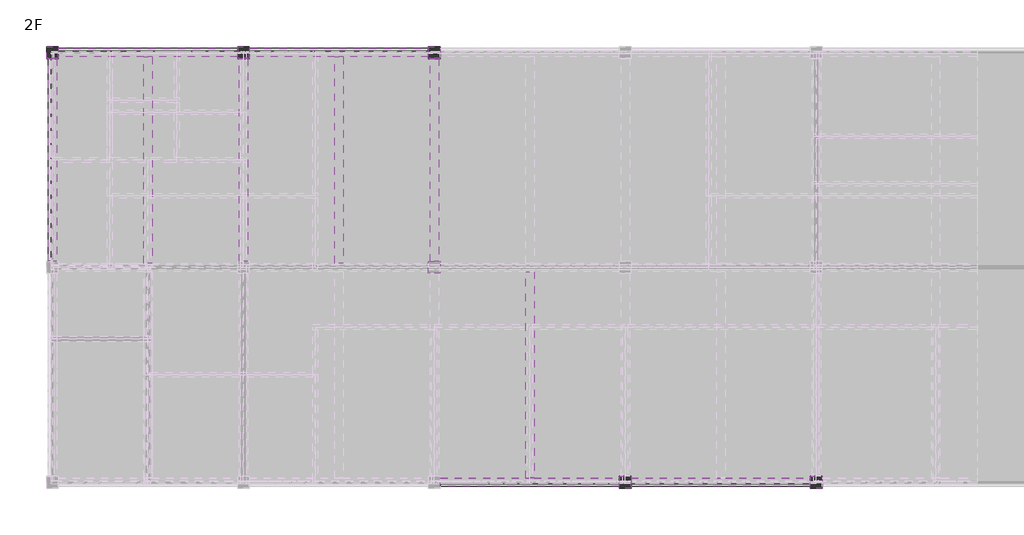
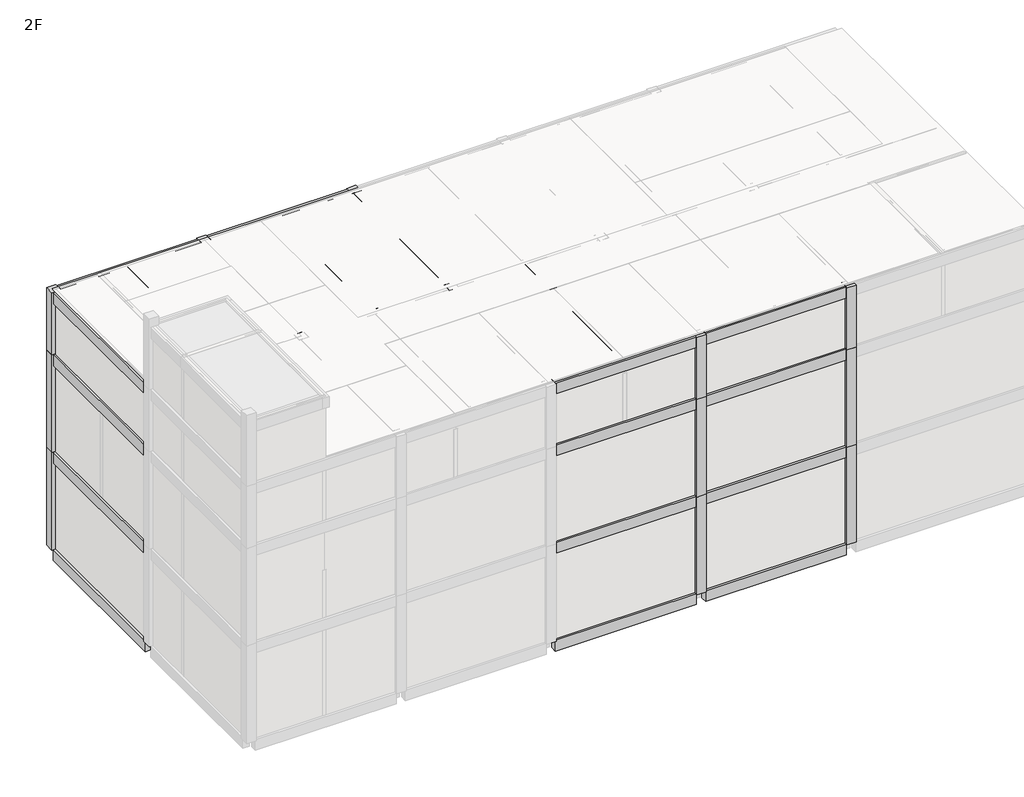
# One storey, part 5 of 7: 40 beams, 17 columns.
"""IFC4 building model written with IfcOpenShell, lengths in millimetres."""

from ifc_helpers import new_model, si_unit, frame, origin, place, context, project, spatial, polyline, outline, extrude, faceted_brep, element, save

model = new_model("IFC4")

# Units and contexts
model_context = context("Model", 3, world=origin())
ifc_project = project(units=[si_unit("LENGTHUNIT", "METRE", prefix="MILLI")], contexts=[model_context])

# Site, building, storey
site = spatial("IfcSite", under=ifc_project)
building = spatial("IfcBuilding", under=site)
storey = spatial("IfcBuildingStorey", under=building, Name="2F", Elevation=3500.0)

# Beams
placement = place(None, origin())
element("IfcBeam", 1, ObjectType="Concrete-Rectangular-Beam : BM111_400x500_RG1", at=placement, inside=storey, context=model_context, shape_type="SweptSolid", body=[
    extrude(outline(polyline([(49284.6521483, 181748.8614395), (49634.6521483, 181748.8614395), (49634.6521483, 173098.8614395), (49284.6521483, 173098.8614395), (49284.6521483, 181748.8614395)])), frame((0.0, 0.0, 2900.0), z_axis=(0.0, 0.0, 1.0), x_axis=(1.0, 0.0, 0.0)), (0.0, 0.0, 1.0), 600.0),
])
element("IfcBeam", 2, ObjectType="Concrete-Rectangular-Beam : BM111_400x500_RG1", at=placement, inside=storey, context=model_context, shape_type="SweptSolid", body=[
    extrude(outline(polyline([(57634.6521483, 173098.8614395), (57284.6521483, 173098.8614395), (57284.6521483, 181748.8614395), (57634.6521483, 181748.8614395), (57634.6521483, 173098.8614395)])), frame((0.0, 0.0, 2900.0), z_axis=(0.0, 0.0, 1.0), x_axis=(1.0, 0.0, 0.0)), (0.0, 0.0, 1.0), 600.0),
])
element("IfcBeam", 3, ObjectType="Concrete-Rectangular-Beam : BM111_400x500_RG1", at=placement, inside=storey, context=model_context, shape_type="SweptSolid", body=[
    extrude(outline(polyline([(65284.6521483, 172748.8614395), (65634.6521483, 172748.8614395), (65634.6521483, 164098.8614395), (65284.6521483, 164098.8614395), (65284.6521483, 172748.8614395)])), frame((0.0, 0.0, 2900.0), z_axis=(0.0, 0.0, 1.0), x_axis=(1.0, 0.0, 0.0)), (0.0, 0.0, 1.0), 600.0),
])
element("IfcBeam", 4, ObjectType="Concrete-Rectangular-Beam : BM111_400x500_RG1", at=placement, inside=storey, context=model_context, shape_type="SweptSolid", body=[
    extrude(outline(polyline([(49284.6521483, 181748.8614395), (49634.6521483, 181748.8614395), (49634.6521483, 173098.8614395), (49284.6521483, 173098.8614395), (49284.6521483, 181748.8614395)])), frame((0.0, 0.0, 8400.0), z_axis=(0.0, 0.0, 1.0), x_axis=(1.0, 0.0, 0.0)), (0.0, 0.0, 1.0), 600.0),
])
element("IfcBeam", 5, ObjectType="Concrete-Rectangular-Beam : BM111_400x500_RG1", at=placement, inside=storey, context=model_context, shape_type="SweptSolid", body=[
    extrude(outline(polyline([(57634.6521483, 173098.8614395), (57284.6521483, 173098.8614395), (57284.6521483, 181748.8614395), (57634.6521483, 181748.8614395), (57634.6521483, 173098.8614395)])), frame((0.0, 0.0, 8400.0), z_axis=(0.0, 0.0, 1.0), x_axis=(1.0, 0.0, 0.0)), (0.0, 0.0, 1.0), 600.0),
])
element("IfcBeam", 6, ObjectType="Concrete-Rectangular-Beam : BM111_400x500_RG1", at=placement, inside=storey, context=model_context, shape_type="SweptSolid", body=[
    extrude(outline(polyline([(65284.6521483, 172748.8614395), (65634.6521483, 172748.8614395), (65634.6521483, 164098.8614395), (65284.6521483, 164098.8614395), (65284.6521483, 172748.8614395)])), frame((0.0, 0.0, 8400.0), z_axis=(0.0, 0.0, 1.0), x_axis=(1.0, 0.0, 0.0)), (0.0, 0.0, 1.0), 600.0),
])
element("IfcBeam", 7, ObjectType="Concrete-Rectangular-Beam : BM111_400x500_RG1", at=placement, inside=storey, context=model_context, shape_type="SweptSolid", body=[
    extrude(outline(polyline([(49284.6521483, 181748.8614395), (49634.6521483, 181748.8614395), (49634.6521483, 173098.8614395), (49284.6521483, 173098.8614395), (49284.6521483, 181748.8614395)])), frame((0.0, 0.0, 13900.0), z_axis=(0.0, 0.0, 1.0), x_axis=(1.0, 0.0, 0.0)), (0.0, 0.0, 1.0), 600.0),
])
element("IfcBeam", 8, ObjectType="Concrete-Rectangular-Beam : BM111_400x500_RG1", at=placement, inside=storey, context=model_context, shape_type="SweptSolid", body=[
    extrude(outline(polyline([(57634.6521483, 173098.8614395), (57284.6521483, 173098.8614395), (57284.6521483, 181748.8614395), (57634.6521483, 181748.8614395), (57634.6521483, 173098.8614395)])), frame((0.0, 0.0, 13900.0), z_axis=(0.0, 0.0, 1.0), x_axis=(1.0, 0.0, 0.0)), (0.0, 0.0, 1.0), 600.0),
])
element("IfcBeam", 9, ObjectType="Concrete-Rectangular-Beam : BM111_400x500_RG1", at=placement, inside=storey, context=model_context, shape_type="SweptSolid", body=[
    extrude(outline(polyline([(65284.6521483, 172748.8614395), (65634.6521483, 172748.8614395), (65634.6521483, 164098.8614395), (65284.6521483, 164098.8614395), (65284.6521483, 172748.8614395)])), frame((0.0, 0.0, 13900.0), z_axis=(0.0, 0.0, 1.0), x_axis=(1.0, 0.0, 0.0)), (0.0, 0.0, 1.0), 600.0),
])
element("IfcBeam", 10, ObjectType="Concrete-Rectangular-Beam : BM111_400x500_RG1", at=placement, inside=storey, context=model_context, shape_type="SweptSolid", body=[
    extrude(outline(polyline([(49284.6521483, 181748.8614395), (49634.6521483, 181748.8614395), (49634.6521483, 173098.8614395), (49284.6521483, 173098.8614395), (49284.6521483, 181748.8614395)])), frame((0.0, 0.0, 17400.0), z_axis=(0.0, 0.0, 1.0), x_axis=(1.0, 0.0, 0.0)), (0.0, 0.0, 1.0), 600.0),
])
element("IfcBeam", 11, ObjectType="Concrete-Rectangular-Beam : BM111_400x500_RG1", at=placement, inside=storey, context=model_context, shape_type="SweptSolid", body=[
    extrude(outline(polyline([(57634.6521483, 173098.8614395), (57284.6521483, 173098.8614395), (57284.6521483, 181748.8614395), (57634.6521483, 181748.8614395), (57634.6521483, 173098.8614395)])), frame((0.0, 0.0, 17400.0), z_axis=(0.0, 0.0, 1.0), x_axis=(1.0, 0.0, 0.0)), (0.0, 0.0, 1.0), 600.0),
])
element("IfcBeam", 12, ObjectType="Concrete-Rectangular-Beam : BM111_400x500_RG1", at=placement, inside=storey, context=model_context, shape_type="SweptSolid", body=[
    extrude(outline(polyline([(65284.6521483, 172748.8614395), (65634.6521483, 172748.8614395), (65634.6521483, 164098.8614395), (65284.6521483, 164098.8614395), (65284.6521483, 172748.8614395)])), frame((0.0, 0.0, 17400.0), z_axis=(0.0, 0.0, 1.0), x_axis=(1.0, 0.0, 0.0)), (0.0, 0.0, 1.0), 600.0),
])
element("IfcBeam", 13, ObjectType="Concrete-Rectangular-Beam : BM111_400x500_RG1", at=placement, inside=storey, context=model_context, shape_type="Brep", body=[
    faceted_brep([(45709.6521483, 182098.8614395, 3500.0), (45709.6521483, 181748.8614395, 3500.0), (49284.6521483, 181748.8614395, 3500.0), (49634.6521483, 181748.8614395, 3500.0), (53209.6521483, 181748.8614395, 3500.0), (53209.6521483, 182098.8614395, 3500.0), (45709.6521483, 181748.8614395, 2900.0), (49284.6521483, 181748.8614395, 2900.0), (49634.6521483, 181748.8614395, 2900.0), (53209.6521483, 181748.8614395, 2900.0), (45709.6521483, 182098.8614395, 2900.0), (53209.6521483, 182098.8614395, 2900.0)], [[[0, 1, 2, 3, 4, 5]], [[1, 6, 7, 8, 9, 4, 3, 2]], [[6, 10, 11, 9, 8, 7]], [[10, 0, 5, 11]], [[1, 0, 10, 6]], [[5, 4, 9, 11]]]),
])
element("IfcBeam", 14, ObjectType="Concrete-Rectangular-Beam : BM111_400x500_RG1", at=placement, inside=storey, context=model_context, shape_type="Brep", body=[
    faceted_brep([(53709.6521483, 182098.8614395, 3500.0), (53709.6521483, 181748.8614395, 3500.0), (57284.6521483, 181748.8614395, 3500.0), (57634.6521483, 181748.8614395, 3500.0), (61209.6521483, 181748.8614395, 3500.0), (61209.6521483, 182098.8614395, 3500.0), (53709.6521483, 181748.8614395, 2900.0), (57284.6521483, 181748.8614395, 2900.0), (57634.6521483, 181748.8614395, 2900.0), (61209.6521483, 181748.8614395, 2900.0), (53709.6521483, 182098.8614395, 2900.0), (61209.6521483, 182098.8614395, 2900.0)], [[[0, 1, 2, 3, 4, 5]], [[1, 6, 7, 8, 9, 4, 3, 2]], [[6, 10, 11, 9, 8, 7]], [[10, 0, 5, 11]], [[1, 0, 10, 6]], [[5, 4, 9, 11]]]),
])
element("IfcBeam", 15, ObjectType="Concrete-Rectangular-Beam : BM111_400x500_RG1", at=placement, inside=storey, context=model_context, shape_type="Brep", body=[
    faceted_brep([(61709.6521483, 164098.8614395, 3500.0), (61709.6521483, 163748.8614395, 3500.0), (69209.6521483, 163748.8614395, 3500.0), (69209.6521483, 164098.8614395, 3500.0), (65634.6521483, 164098.8614395, 3500.0), (65284.6521483, 164098.8614395, 3500.0), (61709.6521483, 163748.8614395, 2900.0), (69209.6521483, 163748.8614395, 2900.0), (61709.6521483, 164098.8614395, 2900.0), (65284.6521483, 164098.8614395, 2900.0), (65634.6521483, 164098.8614395, 2900.0), (69209.6521483, 164098.8614395, 2900.0)], [[[0, 1, 2, 3, 4, 5]], [[1, 6, 7, 2]], [[6, 8, 9, 10, 11, 7]], [[8, 0, 5, 4, 3, 11, 10, 9]], [[1, 0, 8, 6]], [[3, 2, 7, 11]]]),
])
element("IfcBeam", 16, ObjectType="Concrete-Rectangular-Beam : BM111_400x500_RG1", at=placement, inside=storey, context=model_context, shape_type="Brep", body=[
    faceted_brep([(69709.6521483, 164098.8614395, 3500.0), (69709.6521483, 163748.8614395, 3500.0), (77209.6521483, 163748.8614395, 3500.0), (77209.6521483, 164098.8614395, 3500.0), (73634.6521483, 164098.8614395, 3500.0), (73284.6521483, 164098.8614395, 3500.0), (69709.6521483, 163748.8614395, 2900.0), (77209.6521483, 163748.8614395, 2900.0), (69709.6521483, 164098.8614395, 2900.0), (73284.6521483, 164098.8614395, 2900.0), (73634.6521483, 164098.8614395, 2900.0), (77209.6521483, 164098.8614395, 2900.0)], [[[0, 1, 2, 3, 4, 5]], [[1, 6, 7, 2]], [[6, 8, 9, 10, 11, 7]], [[8, 0, 5, 4, 3, 11, 10, 9]], [[1, 0, 8, 6]], [[3, 2, 7, 11]]]),
])
element("IfcBeam", 17, ObjectType="Concrete-Rectangular-Beam : BM111_400x500_RG1", at=placement, inside=storey, context=model_context, shape_type="Brep", body=[
    faceted_brep([(45709.6521483, 182098.8614395, 9000.0), (45709.6521483, 181748.8614395, 9000.0), (49284.6521483, 181748.8614395, 9000.0), (49634.6521483, 181748.8614395, 9000.0), (53209.6521483, 181748.8614395, 9000.0), (53209.6521483, 182098.8614395, 9000.0), (45709.6521483, 181748.8614395, 8400.0), (49284.6521483, 181748.8614395, 8400.0), (49634.6521483, 181748.8614395, 8400.0), (53209.6521483, 181748.8614395, 8400.0), (45709.6521483, 182098.8614395, 8400.0), (53209.6521483, 182098.8614395, 8400.0)], [[[0, 1, 2, 3, 4, 5]], [[1, 6, 7, 8, 9, 4, 3, 2]], [[6, 10, 11, 9, 8, 7]], [[10, 0, 5, 11]], [[1, 0, 10, 6]], [[5, 4, 9, 11]]]),
])
element("IfcBeam", 18, ObjectType="Concrete-Rectangular-Beam : BM111_400x500_RG1", at=placement, inside=storey, context=model_context, shape_type="Brep", body=[
    faceted_brep([(53709.6521483, 182098.8614395, 9000.0), (53709.6521483, 181748.8614395, 9000.0), (57284.6521483, 181748.8614395, 9000.0), (57634.6521483, 181748.8614395, 9000.0), (61209.6521483, 181748.8614395, 9000.0), (61209.6521483, 182098.8614395, 9000.0), (53709.6521483, 181748.8614395, 8400.0), (57284.6521483, 181748.8614395, 8400.0), (57634.6521483, 181748.8614395, 8400.0), (61209.6521483, 181748.8614395, 8400.0), (53709.6521483, 182098.8614395, 8400.0), (61209.6521483, 182098.8614395, 8400.0)], [[[0, 1, 2, 3, 4, 5]], [[1, 6, 7, 8, 9, 4, 3, 2]], [[6, 10, 11, 9, 8, 7]], [[10, 0, 5, 11]], [[1, 0, 10, 6]], [[5, 4, 9, 11]]]),
])
element("IfcBeam", 19, ObjectType="Concrete-Rectangular-Beam : BM111_400x500_RG1", at=placement, inside=storey, context=model_context, shape_type="Brep", body=[
    faceted_brep([(61709.6521483, 164098.8614395, 9000.0), (61709.6521483, 163748.8614395, 9000.0), (69209.6521483, 163748.8614395, 9000.0), (69209.6521483, 164098.8614395, 9000.0), (65634.6521483, 164098.8614395, 9000.0), (65284.6521483, 164098.8614395, 9000.0), (61709.6521483, 163748.8614395, 8400.0), (69209.6521483, 163748.8614395, 8400.0), (61709.6521483, 164098.8614395, 8400.0), (65284.6521483, 164098.8614395, 8400.0), (65634.6521483, 164098.8614395, 8400.0), (69209.6521483, 164098.8614395, 8400.0)], [[[0, 1, 2, 3, 4, 5]], [[1, 6, 7, 2]], [[6, 8, 9, 10, 11, 7]], [[8, 0, 5, 4, 3, 11, 10, 9]], [[1, 0, 8, 6]], [[3, 2, 7, 11]]]),
])
element("IfcBeam", 20, ObjectType="Concrete-Rectangular-Beam : BM111_400x500_RG1", at=placement, inside=storey, context=model_context, shape_type="Brep", body=[
    faceted_brep([(69709.6521483, 164098.8614395, 9000.0), (69709.6521483, 163748.8614395, 9000.0), (77209.6521483, 163748.8614395, 9000.0), (77209.6521483, 164098.8614395, 9000.0), (73634.6521483, 164098.8614395, 9000.0), (73284.6521483, 164098.8614395, 9000.0), (69709.6521483, 163748.8614395, 8400.0), (77209.6521483, 163748.8614395, 8400.0), (69709.6521483, 164098.8614395, 8400.0), (73284.6521483, 164098.8614395, 8400.0), (73634.6521483, 164098.8614395, 8400.0), (77209.6521483, 164098.8614395, 8400.0)], [[[0, 1, 2, 3, 4, 5]], [[1, 6, 7, 2]], [[6, 8, 9, 10, 11, 7]], [[8, 0, 5, 4, 3, 11, 10, 9]], [[1, 0, 8, 6]], [[3, 2, 7, 11]]]),
])
element("IfcBeam", 21, ObjectType="Concrete-Rectangular-Beam : BM111_400x500_RG1", at=placement, inside=storey, context=model_context, shape_type="Brep", body=[
    faceted_brep([(45709.6521483, 182098.8614395, 14500.0), (45709.6521483, 181748.8614395, 14500.0), (49284.6521483, 181748.8614395, 14500.0), (49634.6521483, 181748.8614395, 14500.0), (53209.6521483, 181748.8614395, 14500.0), (53209.6521483, 182098.8614395, 14500.0), (45709.6521483, 181748.8614395, 13900.0), (49284.6521483, 181748.8614395, 13900.0), (49634.6521483, 181748.8614395, 13900.0), (53209.6521483, 181748.8614395, 13900.0), (45709.6521483, 182098.8614395, 13900.0), (53209.6521483, 182098.8614395, 13900.0)], [[[0, 1, 2, 3, 4, 5]], [[1, 6, 7, 8, 9, 4, 3, 2]], [[6, 10, 11, 9, 8, 7]], [[10, 0, 5, 11]], [[1, 0, 10, 6]], [[5, 4, 9, 11]]]),
])
element("IfcBeam", 22, ObjectType="Concrete-Rectangular-Beam : BM111_400x500_RG1", at=placement, inside=storey, context=model_context, shape_type="Brep", body=[
    faceted_brep([(53709.6521483, 182098.8614395, 14500.0), (53709.6521483, 181748.8614395, 14500.0), (57284.6521483, 181748.8614395, 14500.0), (57634.6521483, 181748.8614395, 14500.0), (61209.6521483, 181748.8614395, 14500.0), (61209.6521483, 182098.8614395, 14500.0), (53709.6521483, 181748.8614395, 13900.0), (57284.6521483, 181748.8614395, 13900.0), (57634.6521483, 181748.8614395, 13900.0), (61209.6521483, 181748.8614395, 13900.0), (53709.6521483, 182098.8614395, 13900.0), (61209.6521483, 182098.8614395, 13900.0)], [[[0, 1, 2, 3, 4, 5]], [[1, 6, 7, 8, 9, 4, 3, 2]], [[6, 10, 11, 9, 8, 7]], [[10, 0, 5, 11]], [[1, 0, 10, 6]], [[5, 4, 9, 11]]]),
])
element("IfcBeam", 23, ObjectType="Concrete-Rectangular-Beam : BM111_400x500_RG1", at=placement, inside=storey, context=model_context, shape_type="Brep", body=[
    faceted_brep([(61709.6521483, 164098.8614395, 14500.0), (61709.6521483, 163748.8614395, 14500.0), (69209.6521483, 163748.8614395, 14500.0), (69209.6521483, 164098.8614395, 14500.0), (65634.6521483, 164098.8614395, 14500.0), (65284.6521483, 164098.8614395, 14500.0), (61709.6521483, 163748.8614395, 13900.0), (69209.6521483, 163748.8614395, 13900.0), (61709.6521483, 164098.8614395, 13900.0), (65284.6521483, 164098.8614395, 13900.0), (65634.6521483, 164098.8614395, 13900.0), (69209.6521483, 164098.8614395, 13900.0)], [[[0, 1, 2, 3, 4, 5]], [[1, 6, 7, 2]], [[6, 8, 9, 10, 11, 7]], [[8, 0, 5, 4, 3, 11, 10, 9]], [[1, 0, 8, 6]], [[3, 2, 7, 11]]]),
])
element("IfcBeam", 24, ObjectType="Concrete-Rectangular-Beam : BM111_400x500_RG1", at=placement, inside=storey, context=model_context, shape_type="Brep", body=[
    faceted_brep([(69709.6521483, 164098.8614395, 14500.0), (69709.6521483, 163748.8614395, 14500.0), (77209.6521483, 163748.8614395, 14500.0), (77209.6521483, 164098.8614395, 14500.0), (73634.6521483, 164098.8614395, 14500.0), (73284.6521483, 164098.8614395, 14500.0), (69709.6521483, 163748.8614395, 13900.0), (77209.6521483, 163748.8614395, 13900.0), (69709.6521483, 164098.8614395, 13900.0), (73284.6521483, 164098.8614395, 13900.0), (73634.6521483, 164098.8614395, 13900.0), (77209.6521483, 164098.8614395, 13900.0)], [[[0, 1, 2, 3, 4, 5]], [[1, 6, 7, 2]], [[6, 8, 9, 10, 11, 7]], [[8, 0, 5, 4, 3, 11, 10, 9]], [[1, 0, 8, 6]], [[3, 2, 7, 11]]]),
])
element("IfcBeam", 25, ObjectType="Concrete-Rectangular-Beam : BM111_400x500_RG1", at=placement, inside=storey, context=model_context, shape_type="Brep", body=[
    faceted_brep([(45709.6521483, 182098.8614395, 18000.0), (45709.6521483, 181748.8614395, 18000.0), (49284.6521483, 181748.8614395, 18000.0), (49634.6521483, 181748.8614395, 18000.0), (53209.6521483, 181748.8614395, 18000.0), (53209.6521483, 182098.8614395, 18000.0), (45709.6521483, 181748.8614395, 17400.0), (49284.6521483, 181748.8614395, 17400.0), (49634.6521483, 181748.8614395, 17400.0), (53209.6521483, 181748.8614395, 17400.0), (45709.6521483, 182098.8614395, 17400.0), (53209.6521483, 182098.8614395, 17400.0)], [[[0, 1, 2, 3, 4, 5]], [[1, 6, 7, 8, 9, 4, 3, 2]], [[6, 10, 11, 9, 8, 7]], [[10, 0, 5, 11]], [[1, 0, 10, 6]], [[5, 4, 9, 11]]]),
])
element("IfcBeam", 26, ObjectType="Concrete-Rectangular-Beam : BM111_400x500_RG1", at=placement, inside=storey, context=model_context, shape_type="Brep", body=[
    faceted_brep([(53709.6521483, 182098.8614395, 18000.0), (53709.6521483, 181748.8614395, 18000.0), (57284.6521483, 181748.8614395, 18000.0), (57634.6521483, 181748.8614395, 18000.0), (61209.6521483, 181748.8614395, 18000.0), (61209.6521483, 182098.8614395, 18000.0), (53709.6521483, 181748.8614395, 17400.0), (57284.6521483, 181748.8614395, 17400.0), (57634.6521483, 181748.8614395, 17400.0), (61209.6521483, 181748.8614395, 17400.0), (53709.6521483, 182098.8614395, 17400.0), (61209.6521483, 182098.8614395, 17400.0)], [[[0, 1, 2, 3, 4, 5]], [[1, 6, 7, 8, 9, 4, 3, 2]], [[6, 10, 11, 9, 8, 7]], [[10, 0, 5, 11]], [[1, 0, 10, 6]], [[5, 4, 9, 11]]]),
])
element("IfcBeam", 27, ObjectType="Concrete-Rectangular-Beam : BM111_400x500_RG1", at=placement, inside=storey, context=model_context, shape_type="Brep", body=[
    faceted_brep([(61709.6521483, 164098.8614395, 18000.0), (61709.6521483, 163748.8614395, 18000.0), (69209.6521483, 163748.8614395, 18000.0), (69209.6521483, 164098.8614395, 18000.0), (65634.6521483, 164098.8614395, 18000.0), (65284.6521483, 164098.8614395, 18000.0), (61709.6521483, 163748.8614395, 17400.0), (69209.6521483, 163748.8614395, 17400.0), (61709.6521483, 164098.8614395, 17400.0), (65284.6521483, 164098.8614395, 17400.0), (65634.6521483, 164098.8614395, 17400.0), (69209.6521483, 164098.8614395, 17400.0)], [[[0, 1, 2, 3, 4, 5]], [[1, 6, 7, 2]], [[6, 8, 9, 10, 11, 7]], [[8, 0, 5, 4, 3, 11, 10, 9]], [[1, 0, 8, 6]], [[3, 2, 7, 11]]]),
])
element("IfcBeam", 28, ObjectType="Concrete-Rectangular-Beam : BM111_400x500_RG1", at=placement, inside=storey, context=model_context, shape_type="Brep", body=[
    faceted_brep([(69709.6521483, 164098.8614395, 18000.0), (69709.6521483, 163748.8614395, 18000.0), (77209.6521483, 163748.8614395, 18000.0), (77209.6521483, 164098.8614395, 18000.0), (73634.6521483, 164098.8614395, 18000.0), (73284.6521483, 164098.8614395, 18000.0), (69709.6521483, 163748.8614395, 17400.0), (77209.6521483, 163748.8614395, 17400.0), (69709.6521483, 164098.8614395, 17400.0), (73284.6521483, 164098.8614395, 17400.0), (73634.6521483, 164098.8614395, 17400.0), (77209.6521483, 164098.8614395, 17400.0)], [[[0, 1, 2, 3, 4, 5]], [[1, 6, 7, 2]], [[6, 8, 9, 10, 11, 7]], [[8, 0, 5, 4, 3, 11, 10, 9]], [[1, 0, 8, 6]], [[3, 2, 7, 11]]]),
])
element("IfcBeam", 29, ObjectType="Concrete-Rectangular-Beam : BM111_400x500_RG1", at=placement, inside=storey, context=model_context, shape_type="SweptSolid", body=[
    extrude(outline(polyline([(45284.6521483, 181673.8614395), (45634.6521483, 181673.8614395), (45634.6521483, 173173.8614395), (45284.6521483, 173173.8614395), (45284.6521483, 181673.8614395)])), frame((0.0, 0.0, 2900.0), z_axis=(0.0, 0.0, 1.0), x_axis=(1.0, 0.0, 0.0)), (0.0, 0.0, 1.0), 600.0),
])
element("IfcBeam", 30, ObjectType="Concrete-Rectangular-Beam : BM111_400x500_RG1", at=placement, inside=storey, context=model_context, shape_type="SweptSolid", body=[
    extrude(outline(polyline([(53284.6521483, 181673.8614395), (53634.6521483, 181673.8614395), (53634.6521483, 173173.8614395), (53284.6521483, 173173.8614395), (53284.6521483, 181673.8614395)])), frame((0.0, 0.0, 2900.0), z_axis=(0.0, 0.0, 1.0), x_axis=(1.0, 0.0, 0.0)), (0.0, 0.0, 1.0), 600.0),
])
element("IfcBeam", 31, ObjectType="Concrete-Rectangular-Beam : BM111_400x500_RG1", at=placement, inside=storey, context=model_context, shape_type="SweptSolid", body=[
    extrude(outline(polyline([(61284.6521483, 181673.8614395), (61634.6521483, 181673.8614395), (61634.6521483, 173173.8614395), (61284.6521483, 173173.8614395), (61284.6521483, 181673.8614395)])), frame((0.0, 0.0, 2900.0), z_axis=(0.0, 0.0, 1.0), x_axis=(1.0, 0.0, 0.0)), (0.0, 0.0, 1.0), 600.0),
])
element("IfcBeam", 32, ObjectType="Concrete-Rectangular-Beam : BM111_400x500_RG1", at=placement, inside=storey, context=model_context, shape_type="SweptSolid", body=[
    extrude(outline(polyline([(45284.6521483, 181673.8614395), (45634.6521483, 181673.8614395), (45634.6521483, 173173.8614395), (45284.6521483, 173173.8614395), (45284.6521483, 181673.8614395)])), frame((0.0, 0.0, 8400.0), z_axis=(0.0, 0.0, 1.0), x_axis=(1.0, 0.0, 0.0)), (0.0, 0.0, 1.0), 600.0),
])
element("IfcBeam", 33, ObjectType="Concrete-Rectangular-Beam : BM111_400x500_RG1", at=placement, inside=storey, context=model_context, shape_type="SweptSolid", body=[
    extrude(outline(polyline([(53284.6521483, 181673.8614395), (53634.6521483, 181673.8614395), (53634.6521483, 173173.8614395), (53284.6521483, 173173.8614395), (53284.6521483, 181673.8614395)])), frame((0.0, 0.0, 8400.0), z_axis=(0.0, 0.0, 1.0), x_axis=(1.0, 0.0, 0.0)), (0.0, 0.0, 1.0), 600.0),
])
element("IfcBeam", 34, ObjectType="Concrete-Rectangular-Beam : BM111_400x500_RG1", at=placement, inside=storey, context=model_context, shape_type="SweptSolid", body=[
    extrude(outline(polyline([(61284.6521483, 181673.8614395), (61634.6521483, 181673.8614395), (61634.6521483, 173173.8614395), (61284.6521483, 173173.8614395), (61284.6521483, 181673.8614395)])), frame((0.0, 0.0, 8400.0), z_axis=(0.0, 0.0, 1.0), x_axis=(1.0, 0.0, 0.0)), (0.0, 0.0, 1.0), 600.0),
])
element("IfcBeam", 35, ObjectType="Concrete-Rectangular-Beam : BM111_400x500_RG1", at=placement, inside=storey, context=model_context, shape_type="SweptSolid", body=[
    extrude(outline(polyline([(45284.6521483, 181673.8614395), (45634.6521483, 181673.8614395), (45634.6521483, 173173.8614395), (45284.6521483, 173173.8614395), (45284.6521483, 181673.8614395)])), frame((0.0, 0.0, 13900.0), z_axis=(0.0, 0.0, 1.0), x_axis=(1.0, 0.0, 0.0)), (0.0, 0.0, 1.0), 600.0),
])
element("IfcBeam", 36, ObjectType="Concrete-Rectangular-Beam : BM111_400x500_RG1", at=placement, inside=storey, context=model_context, shape_type="SweptSolid", body=[
    extrude(outline(polyline([(53284.6521483, 181673.8614395), (53634.6521483, 181673.8614395), (53634.6521483, 173173.8614395), (53284.6521483, 173173.8614395), (53284.6521483, 181673.8614395)])), frame((0.0, 0.0, 13900.0), z_axis=(0.0, 0.0, 1.0), x_axis=(1.0, 0.0, 0.0)), (0.0, 0.0, 1.0), 600.0),
])
element("IfcBeam", 37, ObjectType="Concrete-Rectangular-Beam : BM111_400x500_RG1", at=placement, inside=storey, context=model_context, shape_type="SweptSolid", body=[
    extrude(outline(polyline([(61284.6521483, 181673.8614395), (61634.6521483, 181673.8614395), (61634.6521483, 173173.8614395), (61284.6521483, 173173.8614395), (61284.6521483, 181673.8614395)])), frame((0.0, 0.0, 13900.0), z_axis=(0.0, 0.0, 1.0), x_axis=(1.0, 0.0, 0.0)), (0.0, 0.0, 1.0), 600.0),
])
element("IfcBeam", 38, ObjectType="Concrete-Rectangular-Beam : BM111_400x500_RG1", at=placement, inside=storey, context=model_context, shape_type="SweptSolid", body=[
    extrude(outline(polyline([(45284.6521483, 181673.8614395), (45634.6521483, 181673.8614395), (45634.6521483, 173173.8614395), (45284.6521483, 173173.8614395), (45284.6521483, 181673.8614395)])), frame((0.0, 0.0, 17400.0), z_axis=(0.0, 0.0, 1.0), x_axis=(1.0, 0.0, 0.0)), (0.0, 0.0, 1.0), 600.0),
])
element("IfcBeam", 39, ObjectType="Concrete-Rectangular-Beam : BM111_400x500_RG1", at=placement, inside=storey, context=model_context, shape_type="SweptSolid", body=[
    extrude(outline(polyline([(53284.6521483, 181673.8614395), (53634.6521483, 181673.8614395), (53634.6521483, 173173.8614395), (53284.6521483, 173173.8614395), (53284.6521483, 181673.8614395)])), frame((0.0, 0.0, 17400.0), z_axis=(0.0, 0.0, 1.0), x_axis=(1.0, 0.0, 0.0)), (0.0, 0.0, 1.0), 600.0),
])
element("IfcBeam", 40, ObjectType="Concrete-Rectangular-Beam : BM111_400x500_RG1", at=placement, inside=storey, context=model_context, shape_type="SweptSolid", body=[
    extrude(outline(polyline([(61284.6521483, 181673.8614395), (61634.6521483, 181673.8614395), (61634.6521483, 173173.8614395), (61284.6521483, 173173.8614395), (61284.6521483, 181673.8614395)])), frame((0.0, 0.0, 17400.0), z_axis=(0.0, 0.0, 1.0), x_axis=(1.0, 0.0, 0.0)), (0.0, 0.0, 1.0), 600.0),
])

# Columns
element("IfcColumn", 41, ObjectType="Concrete-Rectangular-Column : CL111_500x500", at=placement, inside=storey, context=model_context, shape_type="Brep", body=[
    faceted_brep([(45709.6521483, 182173.8614395, 3500.0), (45709.6521483, 181673.8614395, 3500.0), (45209.6521483, 181673.8614395, 3500.0), (45209.6521483, 182173.8614395, 3500.0), (45709.6521483, 182173.8614395, 9000.0), (45709.6521483, 182098.8614395, 9000.0), (45709.6521483, 181748.8614395, 9000.0), (45709.6521483, 181673.8614395, 9000.0), (45634.6521483, 181673.8614395, 9000.0), (45284.6521483, 181673.8614395, 9000.0), (45209.6521483, 181673.8614395, 9000.0), (45209.6521483, 182173.8614395, 9000.0)], [[[0, 1, 2, 3]], [[4, 5, 6, 7, 1, 0]], [[7, 8, 9, 10, 2, 1]], [[10, 11, 3, 2]], [[11, 4, 0, 3]], [[4, 11, 10, 9, 8, 7, 6, 5]]]),
])
element("IfcColumn", 42, ObjectType="Concrete-Rectangular-Column : CL111_500x500", at=placement, inside=storey, context=model_context, shape_type="Brep", body=[
    faceted_brep([(45709.6521483, 182173.8614395, 9000.0), (45709.6521483, 181673.8614395, 9000.0), (45209.6521483, 181673.8614395, 9000.0), (45209.6521483, 182173.8614395, 9000.0), (45709.6521483, 182173.8614395, 14500.0), (45709.6521483, 182098.8614395, 14500.0), (45709.6521483, 181748.8614395, 14500.0), (45709.6521483, 181673.8614395, 14500.0), (45634.6521483, 181673.8614395, 14500.0), (45284.6521483, 181673.8614395, 14500.0), (45209.6521483, 181673.8614395, 14500.0), (45209.6521483, 182173.8614395, 14500.0)], [[[0, 1, 2, 3]], [[4, 5, 6, 7, 1, 0]], [[7, 8, 9, 10, 2, 1]], [[10, 11, 3, 2]], [[11, 4, 0, 3]], [[4, 11, 10, 9, 8, 7, 6, 5]]]),
])
element("IfcColumn", 43, ObjectType="Concrete-Rectangular-Column : CL111_500x500", at=placement, inside=storey, context=model_context, shape_type="Brep", body=[
    faceted_brep([(45709.6521483, 182173.8614395, 14500.0), (45709.6521483, 181673.8614395, 14500.0), (45209.6521483, 181673.8614395, 14500.0), (45209.6521483, 182173.8614395, 14500.0), (45709.6521483, 182173.8614395, 18000.0), (45709.6521483, 182098.8614395, 18000.0), (45709.6521483, 181748.8614395, 18000.0), (45709.6521483, 181673.8614395, 18000.0), (45634.6521483, 181673.8614395, 18000.0), (45284.6521483, 181673.8614395, 18000.0), (45209.6521483, 181673.8614395, 18000.0), (45209.6521483, 182173.8614395, 18000.0)], [[[0, 1, 2, 3]], [[4, 5, 6, 7, 1, 0]], [[7, 8, 9, 10, 2, 1]], [[10, 11, 3, 2]], [[11, 4, 0, 3]], [[4, 11, 10, 9, 8, 7, 6, 5]]]),
])
element("IfcColumn", 44, ObjectType="Concrete-Rectangular-Column : CL111_500x500", at=placement, inside=storey, context=model_context, shape_type="Brep", body=[
    faceted_brep([(53709.6521483, 182173.8614395, 3500.0), (53709.6521483, 181673.8614395, 3500.0), (53209.6521483, 181673.8614395, 3500.0), (53209.6521483, 182173.8614395, 3500.0), (53709.6521483, 182173.8614395, 9000.0), (53709.6521483, 182098.8614395, 9000.0), (53709.6521483, 181748.8614395, 9000.0), (53709.6521483, 181673.8614395, 9000.0), (53634.6521483, 181673.8614395, 9000.0), (53284.6521483, 181673.8614395, 9000.0), (53209.6521483, 181673.8614395, 9000.0), (53209.6521483, 181748.8614395, 9000.0), (53209.6521483, 182098.8614395, 9000.0), (53209.6521483, 182173.8614395, 9000.0)], [[[0, 1, 2, 3]], [[4, 5, 6, 7, 1, 0]], [[7, 8, 9, 10, 2, 1]], [[10, 11, 12, 13, 3, 2]], [[13, 4, 0, 3]], [[4, 13, 12, 11, 10, 9, 8, 7, 6, 5]]]),
])
element("IfcColumn", 45, ObjectType="Concrete-Rectangular-Column : CL111_500x500", at=placement, inside=storey, context=model_context, shape_type="Brep", body=[
    faceted_brep([(53709.6521483, 182173.8614395, 9000.0), (53709.6521483, 181673.8614395, 9000.0), (53209.6521483, 181673.8614395, 9000.0), (53209.6521483, 182173.8614395, 9000.0), (53709.6521483, 182173.8614395, 14500.0), (53709.6521483, 182098.8614395, 14500.0), (53709.6521483, 181748.8614395, 14500.0), (53709.6521483, 181673.8614395, 14500.0), (53634.6521483, 181673.8614395, 14500.0), (53284.6521483, 181673.8614395, 14500.0), (53209.6521483, 181673.8614395, 14500.0), (53209.6521483, 181748.8614395, 14500.0), (53209.6521483, 182098.8614395, 14500.0), (53209.6521483, 182173.8614395, 14500.0)], [[[0, 1, 2, 3]], [[4, 5, 6, 7, 1, 0]], [[7, 8, 9, 10, 2, 1]], [[10, 11, 12, 13, 3, 2]], [[13, 4, 0, 3]], [[4, 13, 12, 11, 10, 9, 8, 7, 6, 5]]]),
])
element("IfcColumn", 46, ObjectType="Concrete-Rectangular-Column : CL111_500x500", at=placement, inside=storey, context=model_context, shape_type="Brep", body=[
    faceted_brep([(53709.6521483, 182173.8614395, 14500.0), (53709.6521483, 181673.8614395, 14500.0), (53209.6521483, 181673.8614395, 14500.0), (53209.6521483, 182173.8614395, 14500.0), (53709.6521483, 182173.8614395, 18000.0), (53709.6521483, 182098.8614395, 18000.0), (53709.6521483, 181748.8614395, 18000.0), (53709.6521483, 181673.8614395, 18000.0), (53634.6521483, 181673.8614395, 18000.0), (53284.6521483, 181673.8614395, 18000.0), (53209.6521483, 181673.8614395, 18000.0), (53209.6521483, 181748.8614395, 18000.0), (53209.6521483, 182098.8614395, 18000.0), (53209.6521483, 182173.8614395, 18000.0)], [[[0, 1, 2, 3]], [[4, 5, 6, 7, 1, 0]], [[7, 8, 9, 10, 2, 1]], [[10, 11, 12, 13, 3, 2]], [[13, 4, 0, 3]], [[4, 13, 12, 11, 10, 9, 8, 7, 6, 5]]]),
])
element("IfcColumn", 47, ObjectType="Concrete-Rectangular-Column : CL111_500x500", at=placement, inside=storey, context=model_context, shape_type="Brep", body=[
    faceted_brep([(61709.6521483, 182173.8614395, 3500.0), (61709.6521483, 181673.8614395, 3500.0), (61209.6521483, 181673.8614395, 3500.0), (61209.6521483, 182173.8614395, 3500.0), (61709.6521483, 182173.8614395, 9000.0), (61709.6521483, 182098.8614395, 9000.0), (61709.6521483, 181748.8614395, 9000.0), (61709.6521483, 181673.8614395, 9000.0), (61634.6521483, 181673.8614395, 9000.0), (61284.6521483, 181673.8614395, 9000.0), (61209.6521483, 181673.8614395, 9000.0), (61209.6521483, 181748.8614395, 9000.0), (61209.6521483, 182098.8614395, 9000.0), (61209.6521483, 182173.8614395, 9000.0)], [[[0, 1, 2, 3]], [[4, 5, 6, 7, 1, 0]], [[7, 8, 9, 10, 2, 1]], [[10, 11, 12, 13, 3, 2]], [[13, 4, 0, 3]], [[4, 13, 12, 11, 10, 9, 8, 7, 6, 5]]]),
])
element("IfcColumn", 48, ObjectType="Concrete-Rectangular-Column : CL111_500x500", at=placement, inside=storey, context=model_context, shape_type="Brep", body=[
    faceted_brep([(61709.6521483, 182173.8614395, 9000.0), (61709.6521483, 181673.8614395, 9000.0), (61209.6521483, 181673.8614395, 9000.0), (61209.6521483, 182173.8614395, 9000.0), (61709.6521483, 182173.8614395, 14500.0), (61709.6521483, 182098.8614395, 14500.0), (61709.6521483, 181748.8614395, 14500.0), (61709.6521483, 181673.8614395, 14500.0), (61634.6521483, 181673.8614395, 14500.0), (61284.6521483, 181673.8614395, 14500.0), (61209.6521483, 181673.8614395, 14500.0), (61209.6521483, 181748.8614395, 14500.0), (61209.6521483, 182098.8614395, 14500.0), (61209.6521483, 182173.8614395, 14500.0)], [[[0, 1, 2, 3]], [[4, 5, 6, 7, 1, 0]], [[7, 8, 9, 10, 2, 1]], [[10, 11, 12, 13, 3, 2]], [[13, 4, 0, 3]], [[4, 13, 12, 11, 10, 9, 8, 7, 6, 5]]]),
])
element("IfcColumn", 49, ObjectType="Concrete-Rectangular-Column : CL111_500x500", at=placement, inside=storey, context=model_context, shape_type="Brep", body=[
    faceted_brep([(61709.6521483, 182173.8614395, 14500.0), (61709.6521483, 181673.8614395, 14500.0), (61209.6521483, 181673.8614395, 14500.0), (61209.6521483, 182173.8614395, 14500.0), (61709.6521483, 182173.8614395, 18000.0), (61709.6521483, 182098.8614395, 18000.0), (61709.6521483, 181748.8614395, 18000.0), (61709.6521483, 181673.8614395, 18000.0), (61634.6521483, 181673.8614395, 18000.0), (61284.6521483, 181673.8614395, 18000.0), (61209.6521483, 181673.8614395, 18000.0), (61209.6521483, 181748.8614395, 18000.0), (61209.6521483, 182098.8614395, 18000.0), (61209.6521483, 182173.8614395, 18000.0)], [[[0, 1, 2, 3]], [[4, 5, 6, 7, 1, 0]], [[7, 8, 9, 10, 2, 1]], [[10, 11, 12, 13, 3, 2]], [[13, 4, 0, 3]], [[4, 13, 12, 11, 10, 9, 8, 7, 6, 5]]]),
])
element("IfcColumn", 50, ObjectType="Concrete-Rectangular-Column : CL111_500x500", at=placement, inside=storey, context=model_context, shape_type="Brep", body=[
    faceted_brep([(61709.6521483, 173173.8614395, 9000.0), (61709.6521483, 172673.8614395, 9000.0), (61209.6521483, 172673.8614395, 9000.0), (61209.6521483, 173173.8614395, 9000.0), (61709.6521483, 173173.8614395, 14500.0), (61709.6521483, 173098.8614395, 14500.0), (61709.6521483, 172748.8614395, 14500.0), (61709.6521483, 172673.8614395, 14500.0), (61634.6521483, 172673.8614395, 14500.0), (61284.6521483, 172673.8614395, 14500.0), (61209.6521483, 172673.8614395, 14500.0), (61209.6521483, 172748.8614395, 14500.0), (61209.6521483, 173098.8614395, 14500.0), (61209.6521483, 173173.8614395, 14500.0), (61284.6521483, 173173.8614395, 14500.0), (61634.6521483, 173173.8614395, 14500.0)], [[[0, 1, 2, 3]], [[4, 5, 6, 7, 1, 0]], [[7, 8, 9, 10, 2, 1]], [[10, 11, 12, 13, 3, 2]], [[13, 14, 15, 4, 0, 3]], [[4, 15, 14, 13, 12, 11, 10, 9, 8, 7, 6, 5]]]),
])
element("IfcColumn", 51, ObjectType="Concrete-Rectangular-Column : CL111_500x500", at=placement, inside=storey, context=model_context, shape_type="Brep", body=[
    faceted_brep([(61709.6521483, 173173.8614395, 14500.0), (61709.6521483, 172673.8614395, 14500.0), (61209.6521483, 172673.8614395, 14500.0), (61209.6521483, 173173.8614395, 14500.0), (61709.6521483, 173173.8614395, 18000.0), (61709.6521483, 173098.8614395, 18000.0), (61709.6521483, 172748.8614395, 18000.0), (61709.6521483, 172673.8614395, 18000.0), (61634.6521483, 172673.8614395, 18000.0), (61284.6521483, 172673.8614395, 18000.0), (61209.6521483, 172673.8614395, 18000.0), (61209.6521483, 172748.8614395, 18000.0), (61209.6521483, 173098.8614395, 18000.0), (61209.6521483, 173173.8614395, 18000.0), (61284.6521483, 173173.8614395, 18000.0), (61634.6521483, 173173.8614395, 18000.0)], [[[0, 1, 2, 3]], [[4, 5, 6, 7, 1, 0]], [[7, 8, 9, 10, 2, 1]], [[10, 11, 12, 13, 3, 2]], [[13, 14, 15, 4, 0, 3]], [[4, 15, 14, 13, 12, 11, 10, 9, 8, 7, 6, 5]]]),
])
element("IfcColumn", 52, ObjectType="Concrete-Rectangular-Column : CL111_500x500", at=placement, inside=storey, context=model_context, shape_type="Brep", body=[
    faceted_brep([(69709.6521483, 164173.8614395, 3500.0), (69709.6521483, 163673.8614395, 3500.0), (69209.6521483, 163673.8614395, 3500.0), (69209.6521483, 164173.8614395, 3500.0), (69709.6521483, 164173.8614395, 9000.0), (69709.6521483, 164098.8614395, 9000.0), (69709.6521483, 163748.8614395, 9000.0), (69709.6521483, 163673.8614395, 9000.0), (69209.6521483, 163673.8614395, 9000.0), (69209.6521483, 163748.8614395, 9000.0), (69209.6521483, 164098.8614395, 9000.0), (69209.6521483, 164173.8614395, 9000.0), (69284.6521483, 164173.8614395, 9000.0), (69634.6521483, 164173.8614395, 9000.0)], [[[0, 1, 2, 3]], [[4, 5, 6, 7, 1, 0]], [[7, 8, 2, 1]], [[8, 9, 10, 11, 3, 2]], [[11, 12, 13, 4, 0, 3]], [[4, 13, 12, 11, 10, 9, 8, 7, 6, 5]]]),
])
element("IfcColumn", 53, ObjectType="Concrete-Rectangular-Column : CL111_500x500", at=placement, inside=storey, context=model_context, shape_type="Brep", body=[
    faceted_brep([(69709.6521483, 164173.8614395, 9000.0), (69709.6521483, 163673.8614395, 9000.0), (69209.6521483, 163673.8614395, 9000.0), (69209.6521483, 164173.8614395, 9000.0), (69709.6521483, 164173.8614395, 14500.0), (69709.6521483, 164098.8614395, 14500.0), (69709.6521483, 163748.8614395, 14500.0), (69709.6521483, 163673.8614395, 14500.0), (69209.6521483, 163673.8614395, 14500.0), (69209.6521483, 163748.8614395, 14500.0), (69209.6521483, 164098.8614395, 14500.0), (69209.6521483, 164173.8614395, 14500.0), (69284.6521483, 164173.8614395, 14500.0), (69634.6521483, 164173.8614395, 14500.0)], [[[0, 1, 2, 3]], [[4, 5, 6, 7, 1, 0]], [[7, 8, 2, 1]], [[8, 9, 10, 11, 3, 2]], [[11, 12, 13, 4, 0, 3]], [[4, 13, 12, 11, 10, 9, 8, 7, 6, 5]]]),
])
element("IfcColumn", 54, ObjectType="Concrete-Rectangular-Column : CL111_500x500", at=placement, inside=storey, context=model_context, shape_type="Brep", body=[
    faceted_brep([(69709.6521483, 164173.8614395, 14500.0), (69709.6521483, 163673.8614395, 14500.0), (69209.6521483, 163673.8614395, 14500.0), (69209.6521483, 164173.8614395, 14500.0), (69709.6521483, 164173.8614395, 18000.0), (69709.6521483, 164098.8614395, 18000.0), (69709.6521483, 163748.8614395, 18000.0), (69709.6521483, 163673.8614395, 18000.0), (69209.6521483, 163673.8614395, 18000.0), (69209.6521483, 163748.8614395, 18000.0), (69209.6521483, 164098.8614395, 18000.0), (69209.6521483, 164173.8614395, 18000.0), (69284.6521483, 164173.8614395, 18000.0), (69634.6521483, 164173.8614395, 18000.0)], [[[0, 1, 2, 3]], [[4, 5, 6, 7, 1, 0]], [[7, 8, 2, 1]], [[8, 9, 10, 11, 3, 2]], [[11, 12, 13, 4, 0, 3]], [[4, 13, 12, 11, 10, 9, 8, 7, 6, 5]]]),
])
element("IfcColumn", 55, ObjectType="Concrete-Rectangular-Column : CL111_500x500", at=placement, inside=storey, context=model_context, shape_type="Brep", body=[
    faceted_brep([(77709.6521483, 164173.8614395, 3500.0), (77709.6521483, 163673.8614395, 3500.0), (77209.6521483, 163673.8614395, 3500.0), (77209.6521483, 164173.8614395, 3500.0), (77709.6521483, 164173.8614395, 9000.0), (77709.6521483, 164098.8614395, 9000.0), (77709.6521483, 163748.8614395, 9000.0), (77709.6521483, 163673.8614395, 9000.0), (77209.6521483, 163673.8614395, 9000.0), (77209.6521483, 163748.8614395, 9000.0), (77209.6521483, 164098.8614395, 9000.0), (77209.6521483, 164173.8614395, 9000.0), (77284.6521483, 164173.8614395, 9000.0), (77634.6521483, 164173.8614395, 9000.0)], [[[0, 1, 2, 3]], [[4, 5, 6, 7, 1, 0]], [[7, 8, 2, 1]], [[8, 9, 10, 11, 3, 2]], [[11, 12, 13, 4, 0, 3]], [[4, 13, 12, 11, 10, 9, 8, 7, 6, 5]]]),
])
element("IfcColumn", 56, ObjectType="Concrete-Rectangular-Column : CL111_500x500", at=placement, inside=storey, context=model_context, shape_type="Brep", body=[
    faceted_brep([(77709.6521483, 164173.8614395, 9000.0), (77709.6521483, 163673.8614395, 9000.0), (77209.6521483, 163673.8614395, 9000.0), (77209.6521483, 164173.8614395, 9000.0), (77709.6521483, 164173.8614395, 14500.0), (77709.6521483, 164098.8614395, 14500.0), (77709.6521483, 163748.8614395, 14500.0), (77709.6521483, 163673.8614395, 14500.0), (77209.6521483, 163673.8614395, 14500.0), (77209.6521483, 163748.8614395, 14500.0), (77209.6521483, 164098.8614395, 14500.0), (77209.6521483, 164173.8614395, 14500.0), (77284.6521483, 164173.8614395, 14500.0), (77634.6521483, 164173.8614395, 14500.0)], [[[0, 1, 2, 3]], [[4, 5, 6, 7, 1, 0]], [[7, 8, 2, 1]], [[8, 9, 10, 11, 3, 2]], [[11, 12, 13, 4, 0, 3]], [[4, 13, 12, 11, 10, 9, 8, 7, 6, 5]]]),
])
element("IfcColumn", 57, ObjectType="Concrete-Rectangular-Column : CL111_500x500", at=placement, inside=storey, context=model_context, shape_type="Brep", body=[
    faceted_brep([(77709.6521483, 164173.8614395, 14500.0), (77709.6521483, 163673.8614395, 14500.0), (77209.6521483, 163673.8614395, 14500.0), (77209.6521483, 164173.8614395, 14500.0), (77709.6521483, 164173.8614395, 18000.0), (77709.6521483, 164098.8614395, 18000.0), (77709.6521483, 163748.8614395, 18000.0), (77709.6521483, 163673.8614395, 18000.0), (77209.6521483, 163673.8614395, 18000.0), (77209.6521483, 163748.8614395, 18000.0), (77209.6521483, 164098.8614395, 18000.0), (77209.6521483, 164173.8614395, 18000.0), (77284.6521483, 164173.8614395, 18000.0), (77634.6521483, 164173.8614395, 18000.0)], [[[0, 1, 2, 3]], [[4, 5, 6, 7, 1, 0]], [[7, 8, 2, 1]], [[8, 9, 10, 11, 3, 2]], [[11, 12, 13, 4, 0, 3]], [[4, 13, 12, 11, 10, 9, 8, 7, 6, 5]]]),
])

save(model, "model.ifc")

# Revit data of these elements
# Type "Concrete-Rectangular-Beam : BM111_400x500_RG1"
#   중앙부 하부근 = "3-D20"
#   중앙부 상부근 = "3-D20"
#   중앙부 보조근 = ""
#   중앙부 늑근 = "2-D10 @200"
#   외단부 하부근 = "3-D20"
#   외단부 상부근 = "3-D20"
#   외단부 보조근 = ""
#   외단부 늑근 = "2-D10 @100"
#   부호 = "RG1"
#   내단부 하부근 = "3-D20"
#   내단부 상부근 = "3-D20"
#   내단부 보조근 = ""
#   내단부 늑근 = "2-D10 @100"
#   ALL 하부근 = ""
#   ALL 상부근 = ""
#   ALL 보조근 = ""
#   ALL 늑근 = ""
#   Width = 400 mm
#   Height = 500 mm
#   Length [instance default] = 1524 mm
#   Structural Material [instance default] = 콘크리트 - 현장타설 콘크리트
#   hec_material3 [instance default] = none
#   hec_material2 [instance default] = none
#   hec_material1 [instance default] = none
#   Assembly Code = ""
# Type "Concrete-Rectangular-Column : CL111_500x500"
#   Description = "UG 철골 기둥용 Pedestal"
#   b = 500 mm
#   h = 500 mm
#   hec_material3 [instance default] = none
#   hec_material2 [instance default] = A03AE056-00001_Bitumen/Bituminous/Asphalt Coating
#   hec_material1 [instance default] = A03AC035-00001_Form Work (3 times in use)_Flat
#   Structural Material [instance default] = A03AC032-00007_Structural Concrete_Type1_25MPa-30Mpa
# Elements 1, 2, 3, 4, 5, 6, 7, 8, 9, 10, 11, 12, 13, 14, 15, 16, 17, 18, 19, 20, 21, 22, 23, 24, 25, 26, 27, 28, 29, 30, 31, 32, 33, 34, 35, 36, 37, 38, 39, 40 (IfcBeam, "Concrete-Rectangular-Beam : BM111_400x500_RG1")
#   Comments = ""
#   hec_material3 = none
#   hec_material2 = none
#   hec_material1 = none
#   Structural Material = 콘크리트 - 현장타설 콘크리트
#   Phase Created = New Construction
#   Materials on its faces: "콘크리트 - 현장타설 콘크리트"
# Elements 41, 42, 43, 44, 45, 46, 47, 48, 49, 50, 51, 52, 53, 54, 55, 56, 57 (IfcColumn, "Concrete-Rectangular-Column : CL111_500x500")
#   Comments = ""
#   hec_material3 = none
#   hec_material2 = none
#   hec_material1 = none
#   Structural Material = 콘크리트 - 현장타설 콘크리트
#   Phase Created = New Construction
#   Materials on its faces: "콘크리트 - 현장타설 콘크리트"
# Materials
#   "콘크리트 - 현장타설 콘크리트": class "콘크리트", colour RGB 192 192 192, transparency 0
#   "A03AE056-00001_Bitumen/Bituminous/Asphalt Coating": class "Generic", colour RGB 17 17 17, transparency 0, Description = "Damp-proofing", W00) Work Master Code = "A03AE056-00001", W01) Work Master_Lv1 = "Concrete Work", W02) Work Master_Lv2 = "Concrete Protective Coating (U/G)", W03) Work Master_Spec.1 = "Bitumen/Bituminous/Asphalt Coating", Cost = 0
#   "A03AC035-00001_Form Work (3 times in use)_Flat": class "Wood", colour RGB 149 120 74, transparency 0, Description = "Plywood", W00) Work Master Code = "A03AC035-00001", W01) Work Master_Lv1 = "Concrete Work", W02) Work Master_Lv2 = "Substructure Work", W03) Work Master_Spec.1 = "Form Work (3 times in use)", W04) Work Master_Spec.2 = "Flat Form", W05) Work Master_Spec.3 = "Dressed Lumber, Plywood or Steel Form(Wood Planks are not Allowed) incl. Chamfer", Cost = 0
#   "A03AC032-00007_Structural Concrete_Type1_25MPa-30Mpa": class "Concrete", colour RGB 176 176 176, transparency 0, Keynote = "09910.A1", Description = "Reinf. Conc.", W00) Work Master Code = "A03AC032-00007", W01) Work Master_Lv1 = "Concrete Work", W02) Work Master_Lv2 = "Substructure Work", W03) Work Master_Spec.1 = "Structural Concrete", W04) Work Master_Spec.2 = "Cement Type-1", W05) Work Master_Spec.3 = "25MPa < F'c (Cylinder Strength) ≤ 30MPa", Cost = 0
# Room at (79959.652, 167173.861) mm, phase "New Construction", upper offset 2700 mm, lower offset 0 mm
#   Department = "AR"
#   Base Finish = "WK3"
#   Ceiling Finish = "CL3"
#   Wall Finish = "IW5"
#   Floor Finish = "FL2"
#   Number = "4.5"
#   Name = "Office-1"
#   Interior Finish = "IW5..N/A..N/A,,WK3..N/A,,FL2..N/A,,CL3..N/A"
#   Exterior Finish = "RF1..N/A,,EW2..N/A..N/A"
# Room at (84959.652, 167173.861) mm, phase "New Construction", upper offset 3500 mm, lower offset 0 mm
#   Department = "FF"
#   Base Finish = "WK1"
#   Ceiling Finish = ""
#   Wall Finish = "IW5"
#   Floor Finish = "FL1"
#   Number = "4.6"
#   Name = "Fire Gas Room"
#   Interior Finish = "IW5..N/A..N/A,,WK1..N/A,,FL1..N/A,,N/A..N/A"
#   Exterior Finish = "RF1..N/A,,EW2..N/A..N/A"
# Room at (78709.652, 174423.861) mm, phase "New Construction", upper offset 2700 mm, lower offset 0 mm
#   Department = "AR"
#   Base Finish = "WK3"
#   Ceiling Finish = "CL3"
#   Wall Finish = "IW5"
#   Floor Finish = "FL2"
#   Number = "4.7"
#   Name = "Document Room"
#   Interior Finish = "IW5..N/A..N/A,,WK3..N/A,,FL2..N/A,,CL3..N/A"
#   Exterior Finish = "RF1..N/A,,N/A..N/A..N/A"
# Room at (58959.652, 167173.861) mm, phase "New Construction", upper offset 2700 mm, lower offset 0 mm
#   Department = "AR"
#   Base Finish = "WK3"
#   Ceiling Finish = "CL3"
#   Wall Finish = "IW5"
#   Floor Finish = "FL2"
#   Number = "4.8"
#   Name = "Storage"
#   Interior Finish = "IW5..N/A..N/A,,WK3..N/A,,FL2..N/A,,CL3..N/A"
#   Exterior Finish = "RF1..N/A,,EW1..N/A..N/A"
# Room at (52959.652, 166173.861) mm, phase "New Construction", upper offset 2700 mm, lower offset 0 mm
#   Department = "AR"
#   Base Finish = "WK3"
#   Ceiling Finish = "CL3"
#   Wall Finish = "IW5"
#   Floor Finish = "FL2"
#   Number = "4.9"
#   Name = "Break Room"
#   Interior Finish = "IW5..N/A..N/A,,WK3..N/A,,FL2..N/A,,CL3..N/A"
#   Exterior Finish = "RF1..N/A,,EW2..N/A..N/A"
# Room at (50659.652, 177673.861) mm, phase "New Construction", upper offset 2700 mm, lower offset 0 mm
#   Department = "AR"
#   Base Finish = ""
#   Ceiling Finish = "CL4"
#   Wall Finish = "IW3"
#   Floor Finish = "FL3"
#   Number = "4.10"
#   Name = "Toilet"
#   Interior Finish = "IW3..N/A..N/A,,N/A..N/A,,FL3..N/A,,CL4..N/A"
#   Exterior Finish = "RF1..N/A,,N/A..N/A..N/A"
# Room at (50659.652, 180673.861) mm, phase "New Construction", upper offset 2700 mm, lower offset 0 mm
#   Department = "AR"
#   Base Finish = ""
#   Ceiling Finish = "CL4"
#   Wall Finish = "IW3"
#   Floor Finish = "FL3"
#   Number = "4.11"
#   Name = "Shower"
#   Interior Finish = "IW3..N/A..N/A,,N/A..N/A,,FL3..N/A,,CL4..N/A"
#   Exterior Finish = "RF1..N/A,,EW2..N/A..N/A"
# Room at (61459.652, 177423.861) mm, phase "New Construction", upper offset 5500 mm, lower offset 0 mm
#   Department = "CI"
#   Base Finish = "WK1"
#   Ceiling Finish = "CL1"
#   Wall Finish = "IW5"
#   Floor Finish = "FL1"
#   Number = "2.0"
#   Name = "Electrical Room-1"
#   Interior Finish = "IW5..N/A..N/A,,WK1..N/A,,FL1..N/A,,CL1..N/A"
#   Exterior Finish = "N/A..N/A,,EW1..EW2..N/A"
# Room at (70459.652, 168423.861) mm, phase "New Construction", upper offset 5500 mm, lower offset 0 mm
#   Department = "EL"
#   Base Finish = "WK1"
#   Ceiling Finish = "CL1"
#   Wall Finish = "IW5"
#   Floor Finish = "FL1"
#   Number = "2.1"
#   Name = "Electrical Room-2"
#   Interior Finish = "IW5..N/A..N/A,,WK1..N/A,,FL1..N/A,,CL1..N/A"
#   Exterior Finish = "N/A..N/A,,EW1..EW2..N/A"
# Room at (82459.652, 177423.861) mm, phase "New Construction", upper offset 5500 mm, lower offset 0 mm
#   Department = "AR"
#   Base Finish = "WK1"
#   Ceiling Finish = "CL1"
#   Wall Finish = "IW5"
#   Floor Finish = "FL1"
#   Number = "2.2"
#   Name = "Electrical Room (GIS)"
#   Interior Finish = "IW5..N/A..N/A,,WK1..N/A,,FL1..N/A,,CL1..N/A"
#   Exterior Finish = "N/A..N/A,,EW1..EW2..N/A"
# Room at (51459.652, 168423.861) mm, phase "New Construction", upper offset 2700 mm, lower offset 0 mm
#   Department = "AR"
#   Base Finish = "WK3"
#   Ceiling Finish = "CL3"
#   Wall Finish = "IW5"
#   Floor Finish = "FL2"
#   Number = "2.3"
#   Name = "Lobby"
#   Interior Finish = "IW5..N/A..N/A,,WK3..N/A,,FL2..N/A,,CL3..N/A"
#   Exterior Finish = "N/A..N/A,,EW2..N/A..N/A"
# Room at (47459.652, 171423.861) mm, phase "New Construction", upper offset 5500 mm, lower offset 0 mm
#   Department = "PATHV2"
#   Base Finish = ""
#   Ceiling Finish = ""
#   Wall Finish = ""
#   Floor Finish = ""
#   Number = "2.4"
#   Name = "Elevator"
#   Interior Finish = "N/A..N/A..N/A,,N/A..N/A,,N/A..N/A,,N/A..N/A"
#   Exterior Finish = "N/A..N/A,,EW2..N/A..N/A"
# Room at (47459.652, 166923.861) mm, phase "New Construction", upper offset 5500 mm, lower offset 0 mm
#   Department = "PATHV1"
#   Base Finish = "WK3"
#   Ceiling Finish = "CL1"
#   Wall Finish = "IW5"
#   Floor Finish = "FL2"
#   Number = "2.5"
#   Name = "Staircase"
#   Interior Finish = "IW5..N/A..N/A,,WK3..N/A,,FL2..N/A,,CL1..N/A"
#   Exterior Finish = "N/A..N/A,,EW2..N/A..N/A"
# Room at (65459.652, 177423.861) mm, phase "New Construction", upper offset 3400 mm, lower offset 0 mm
#   Department = "CI"
#   Base Finish = ""
#   Ceiling Finish = "CL3"
#   Wall Finish = "IW5"
#   Floor Finish = "FL5"
#   Number = "3.0"
#   Name = "Central Control Room"
#   Interior Finish = "IW5..N/A..N/A,,N/A..N/A,,FL5..N/A,,CL3..N/A"
#   Exterior Finish = "N/A..N/A,,EW1..N/A..N/A"
# Room at (65459.652, 168423.861) mm, phase "New Construction", upper offset 3000 mm, lower offset 0 mm
#   Department = "CI"
#   Base Finish = ""
#   Ceiling Finish = "CL3"
#   Wall Finish = "IW5"
#   Floor Finish = "FL5"
#   Number = "3.1"
#   Name = "Electronic Room"
#   Interior Finish = "IW5..N/A..N/A,,N/A..N/A,,FL5..N/A,,CL3..N/A"
#   Exterior Finish = "N/A..N/A,,EW1..N/A..N/A"
# Room at (80959.652, 180173.861) mm, phase "New Construction", upper offset 2700 mm, lower offset 0 mm
#   Department = "AR"
#   Base Finish = ""
#   Ceiling Finish = "CL3"
#   Wall Finish = "IW5"
#   Floor Finish = "FL5"
#   Number = "3.2"
#   Name = "Computer Room"
#   Interior Finish = "IW5..N/A..N/A,,N/A..N/A,,FL5..N/A,,CL3..N/A"
#   Exterior Finish = "N/A..N/A,,EW2..N/A..N/A"
# Room at (82459.652, 168423.861) mm, phase "New Construction", upper offset 5500 mm, lower offset 0 mm
#   Department = "EL"
#   Base Finish = ""
#   Ceiling Finish = "CL3"
#   Wall Finish = "IW5"
#   Floor Finish = "FL5"
#   Number = "3.3"
#   Name = "Electrical Room -3"
#   Interior Finish = "IW5..N/A..N/A,,N/A..N/A,,FL5,,CL3..N/A"
#   Exterior Finish = "N/A..N/A,,EW2..N/A..N/A"
# Room at (80959.652, 174673.861) mm, phase "New Construction", upper offset 2700 mm, lower offset 0 mm
#   Department = "CI"
#   Base Finish = ""
#   Ceiling Finish = "CL3"
#   Wall Finish = "IW5"
#   Floor Finish = "FL5"
#   Number = "3.4"
#   Name = "Communication Room"
#   Interior Finish = "IW5..N/A..N/A,,N/A..N/A,,FL5..N/A,,CL3..N/A"
#   Exterior Finish = "N/A..N/A,,N/A..N/A..N/A"
# Room at (46659.652, 179673.861) mm, phase "New Construction", upper offset 5500 mm, lower offset 0 mm
#   Department = "PATHV3"
#   Base Finish = ""
#   Ceiling Finish = ""
#   Wall Finish = ""
#   Floor Finish = ""
#   Number = "3.5"
#   Name = "Duct Shaft"
#   Interior Finish = "N/A..N/A..N/A,,N/A..N/A,,N/A..N/A,,N/A..N/A"
#   Exterior Finish = "N/A..N/A,,EW2..N/A..N/A"
# Room at (47459.652, 175173.861) mm, phase "New Construction", upper offset 2700 mm, lower offset 0 mm
#   Department = "AR"
#   Base Finish = ""
#   Ceiling Finish = "CL4"
#   Wall Finish = "IW3"
#   Floor Finish = "FL3"
#   Number = "3.6"
#   Name = "Toilet (M)"
#   Interior Finish = "IW3..N/A..N/A,,N/A..N/A,,FL3..N/A,,CL4..N/A"
#   Exterior Finish = "N/A..N/A,,EW2..N/A..N/A"
# Room at (52059.652, 179673.861) mm, phase "New Construction", upper offset 2700 mm, lower offset 0 mm
#   Department = "AR"
#   Base Finish = ""
#   Ceiling Finish = "CL4"
#   Wall Finish = "IW3"
#   Floor Finish = "FL3"
#   Number = "3.7"
#   Name = "Toilet"
#   Interior Finish = "IW3..N/A..N/A,,N/A..N/A,,FL3..N/A,,CL4..N/A"
#   Exterior Finish = "N/A..N/A,,EW2..N/A..N/A"
# Room at (49259.652, 180923.861) mm, phase "New Construction", upper offset 2700 mm, lower offset 0 mm
#   Department = "AR"
#   Base Finish = ""
#   Ceiling Finish = "CL4"
#   Wall Finish = "IW3"
#   Floor Finish = "FL3"
#   Number = "3.8"
#   Name = "Shower"
#   Interior Finish = "IW3..N/A..N/A,,N/A..N/A,,FL3..N/A,,CL4..N/A"
#   Exterior Finish = "N/A..N/A,,EW2..N/A..N/A"
# Room at (49259.652, 178673.861) mm, phase "New Construction", upper offset 2700 mm, lower offset 0 mm
#   Department = "AR"
#   Base Finish = "WK3"
#   Ceiling Finish = "CL3"
#   Wall Finish = "IW5"
#   Floor Finish = "FL2"
#   Number = "3.9"
#   Name = "Locker(F)"
#   Interior Finish = "IW5..N/A..N/A,,WK3..N/A,,FL2..N/A,,CL3..N/A"
#   Exterior Finish = "N/A..N/A,,N/A..N/A..N/A"
# Room at (47459.652, 171423.861) mm, phase "New Construction", upper offset 5500 mm, lower offset 0 mm
#   Department = "PATHV2"
#   Base Finish = ""
#   Ceiling Finish = ""
#   Wall Finish = ""
#   Floor Finish = ""
#   Number = "3.10"
#   Name = "Elevator"
#   Interior Finish = "N/A..N/A..N/A,,N/A..N/A,,N/A..N/A,,N/A..N/A"
#   Exterior Finish = "N/A..N/A,,EW2..N/A..N/A"
# Room at (47459.652, 166923.861) mm, phase "New Construction", upper offset 2700 mm, lower offset 0 mm
#   Department = "PATHV1"
#   Base Finish = "WK3"
#   Ceiling Finish = "CL1"
#   Wall Finish = "IW5"
#   Floor Finish = "FL2"
#   Number = "3.11"
